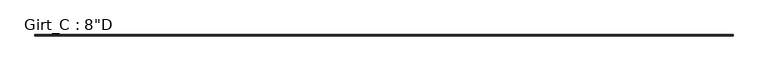
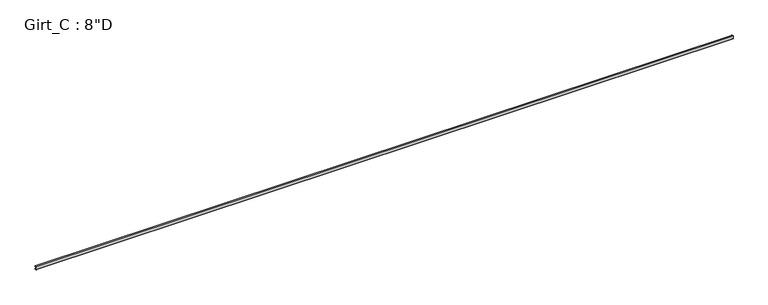
"""IFC4 building model written with IfcOpenShell, lengths in millimetres: beam geometry."""

from ifc_helpers import new_model, si_unit, point, frame, frame_2d, origin, place, context, project, spatial, polyline, circle_curve, trimmed, segment, composite_curve, outline, extrude, source, transform, mapped, element, save


def beam_21065925(model_context):
    return source(origin(), model_context, "Body", "SweptSolid", [
        extrude(outline(composite_curve([segment(polyline([(63.5, 101.6), (75.745104, 87.0068534), (73.6169367, 85.221109), (62.204539, 98.821875), (3.3005807, 98.821875)]), True, "CONTINUOUS"), segment(trimmed(circle_curve(frame_2d((3.3741066, 96.8381931)), 1.9850441), [point((3.3005807, 98.821875))], [point((1.3890625, 96.8381931))], True, "CARTESIAN"), True, "CONTINUOUS"), segment(polyline([(1.3890625, 96.8381931), (1.3890625, -96.8389339)]), True, "CONTINUOUS"), segment(trimmed(circle_curve(frame_2d((3.3748024, -96.8389339)), 1.9857399), [point((1.3890625, -96.8389339))], [point((3.2694106, -98.821875))], True, "CARTESIAN"), True, "CONTINUOUS"), segment(polyline([(3.2694106, -98.821875), (62.204539, -98.821875), (73.6169367, -85.221109), (75.745104, -87.0068534), (63.5, -101.6), (3.3734375, -101.6)]), True, "CONTINUOUS"), segment(trimmed(circle_curve(frame_2d((3.3734375, -96.8375)), 4.7625), [point((3.3734375, -101.6))], [point((-1.3890625, -96.8375))], False, "CARTESIAN"), True, "CONTINUOUS"), segment(polyline([(-1.3890625, -96.8375), (-1.3890625, 96.8375)]), True, "CONTINUOUS"), segment(trimmed(circle_curve(frame_2d((3.3734375, 96.8375)), 4.7625), [point((-1.3890625, 96.8375))], [point((3.3734375, 101.6))], False, "CARTESIAN"), True, "CONTINUOUS"), segment(polyline([(3.3734375, 101.6), (63.5, 101.6)]), True, "CONTINUOUS")], self_intersect=False)), frame((-20891.5, 0.0, 0.0), z_axis=(1.0, 0.0, 0.0), x_axis=(0.0, 1.0, 0.0)), (0.0, 0.0, 1.0), 41643.3),
    ])


if __name__ == "__main__":
    model = new_model("IFC4")
    model_context = context("Model", 3, world=origin())
    ifc_project = project(units=[si_unit("LENGTHUNIT", "METRE", prefix="MILLI")], contexts=[model_context])
    site = spatial("IfcSite", under=ifc_project)
    building = spatial("IfcBuilding", under=site)
    placement = place(None, origin())
    beam_shape = beam_21065925(model_context)
    element("IfcBeam", 1, ObjectType="Girt_C : 8\"D", at=placement, inside=building, context=model_context, shape_type="MappedRepresentation", body=[
        mapped(beam_shape, transform((0.0, 0.0, 0.0), x_axis=(1.0, 0.0, 0.0), y_axis=(0.0, 1.0, 0.0), z_axis=(0.0, 0.0, 1.0))),
    ])
    save(model, "model.ifc")

# Revit data of these elements
# Type "Girt_C : 8\"D"
#   Web_Thickness = 0' - 0 7/64"
#   Length [instance default] = 10' - 0"
#   Leg_1 = 0' - 2 1/2"
#   Height = 0' - 8"
#   Structural Material [instance default] = none
# Element 1 (IfcBeam, "Girt_C : 8\"D")
#   Materials on its faces: "Steel"
# Materials
#   "Steel": class "Metal", colour RGB 118 118 114, transparency 0, Description = "Steel, mill finish", Cost = 0
